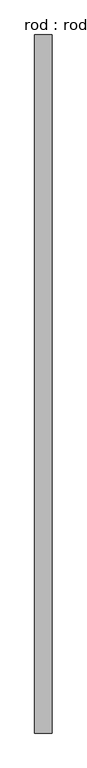
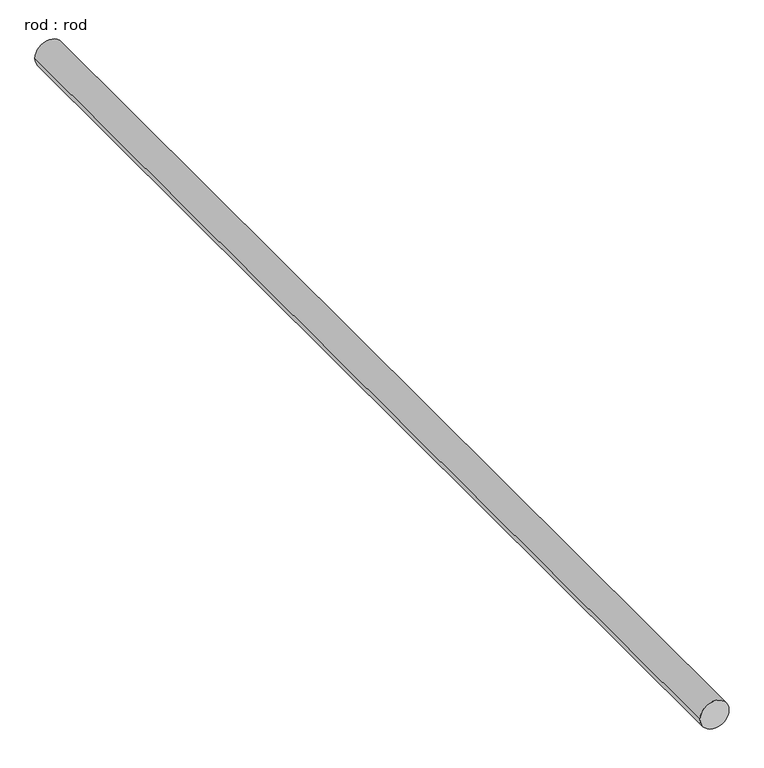
"""IFC4 building model written with IfcOpenShell, lengths in millimetres: proxy geometry, rod : rod."""

from ifc_helpers import new_model, si_unit, point, frame, frame_2d, origin, place, context, project, spatial, circle_curve, trimmed, segment, composite_curve, outline, extrude, source, transform, mapped, element, save


def rod_rod_f7d01b97(model_context):
    return source(origin(), model_context, "Body", "SweptSolid", [
        extrude(outline(composite_curve([segment(trimmed(circle_curve(frame_2d((0.0108462, 0.0)), 200.0), [point((0.0108462, 200.0))], [point((0.0108462, -200.0))], False, "CARTESIAN"), True, "CONTINUOUS"), segment(trimmed(circle_curve(frame_2d((0.0108462, 0.0)), 200.0), [point((0.0108462, -200.0))], [point((0.0108462, 200.0))], False, "CARTESIAN"), True, "CONTINUOUS")], self_intersect=False)), frame((0.0, -3858.0087848, 0.0), z_axis=(0.0, 1.0, 0.0), x_axis=(0.0, 0.0, 1.0)), (0.0, 0.0, 1.0), 15901.4748004),
    ])


if __name__ == "__main__":
    model = new_model("IFC4")
    model_context = context("Model", 3, world=origin())
    ifc_project = project(units=[si_unit("LENGTHUNIT", "METRE", prefix="MILLI")], contexts=[model_context])
    site = spatial("IfcSite", under=ifc_project)
    building = spatial("IfcBuilding", under=site)
    placement = place(None, origin())
    rod_rod_shape = rod_rod_f7d01b97(model_context)
    element("IfcBuildingElementProxy", 1, Name="rod : rod", ObjectType="rod : rod", at=placement, inside=building, context=model_context, shape_type="MappedRepresentation", body=[
        mapped(rod_rod_shape, transform((0.0, 0.0, 0.0), x_axis=(1.0, 0.0, 0.0), y_axis=(0.0, 1.0, 0.0), z_axis=(0.0, 0.0, 1.0))),
    ])
    save(model, "model.ifc")

# Revit data of these elements
# Type "rod : rod"
#   Default Elevation = 0
